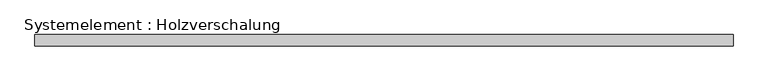
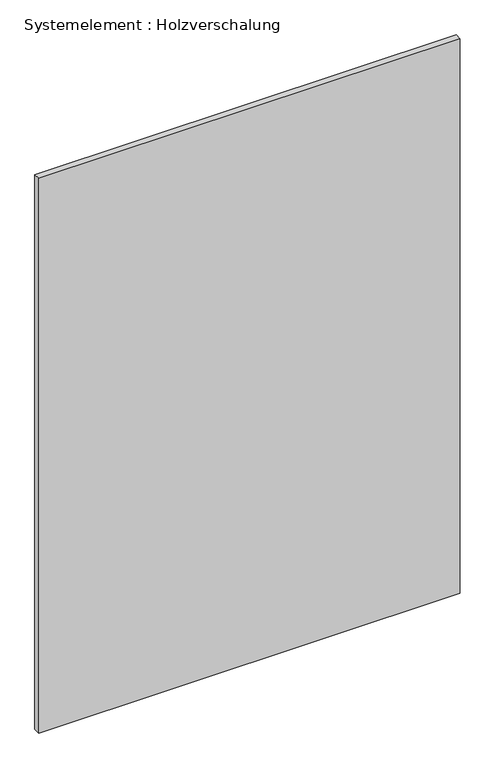
"""IFC4 building model written with IfcOpenShell, lengths in millimetres: plate geometry, Systemelement : Holzverschalung."""

from ifc_helpers import new_model, si_unit, origin, origin_with_axes, place, context, project, spatial, polyline, outline, extrude, source, transform, mapped, element, save


def systemelement_holzverschalung_cedf78a1(model_context):
    return source(origin(), model_context, "Body", "SweptSolid", [
        extrude(outline(polyline([(1566.4783809, -25.0), (-1566.4783809, -25.0), (-1566.4783809, 25.0), (1566.4783809, 25.0), (1566.4783809, -25.0)])), origin_with_axes(), (0.0, 0.0, 1.0), 4356.6788019),
    ])


if __name__ == "__main__":
    model = new_model("IFC4")
    model_context = context("Model", 3, world=origin())
    ifc_project = project(units=[si_unit("LENGTHUNIT", "METRE", prefix="MILLI")], contexts=[model_context])
    site = spatial("IfcSite", under=ifc_project)
    building = spatial("IfcBuilding", under=site)
    placement = place(None, origin())
    systemelement_holzverschalung_shape = systemelement_holzverschalung_cedf78a1(model_context)
    element("IfcPlate", 1, ObjectType="Systemelement : Holzverschalung", at=placement, inside=building, context=model_context, shape_type="MappedRepresentation", body=[
        mapped(systemelement_holzverschalung_shape, transform((0.0, 0.0, 0.0), x_axis=(1.0, 0.0, 0.0), y_axis=(0.0, 1.0, 0.0), z_axis=(0.0, 0.0, 1.0))),
    ])
    save(model, "model.ifc")

# Revit data of these elements
# Type "Systemelement : Holzverschalung"
#   Construction Type Id = "MDOOR"
#   Analytic Construction = "Metall"
#   Visual Light Transmittance = 0
#   Solar Heat Gain Coefficient = 0
#   Heat Transfer Coefficient (U) = 3.7021 W/(m²·K)
# Element 1 (IfcPlate, "Systemelement : Holzverschalung")
#   Materials on its faces: "Fassade - Holzverschalung"
# Materials
#   "Fassade - Holzverschalung": class "Holz", colour RGB 216 169 114, transparency 0, Cost = 0
